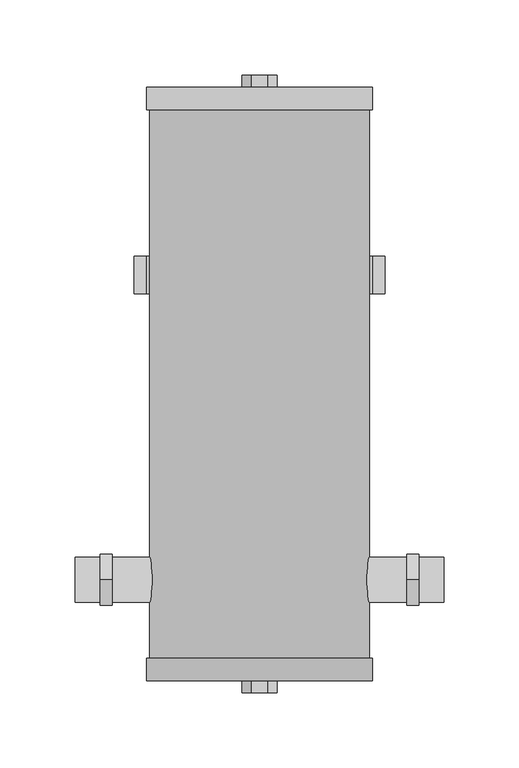
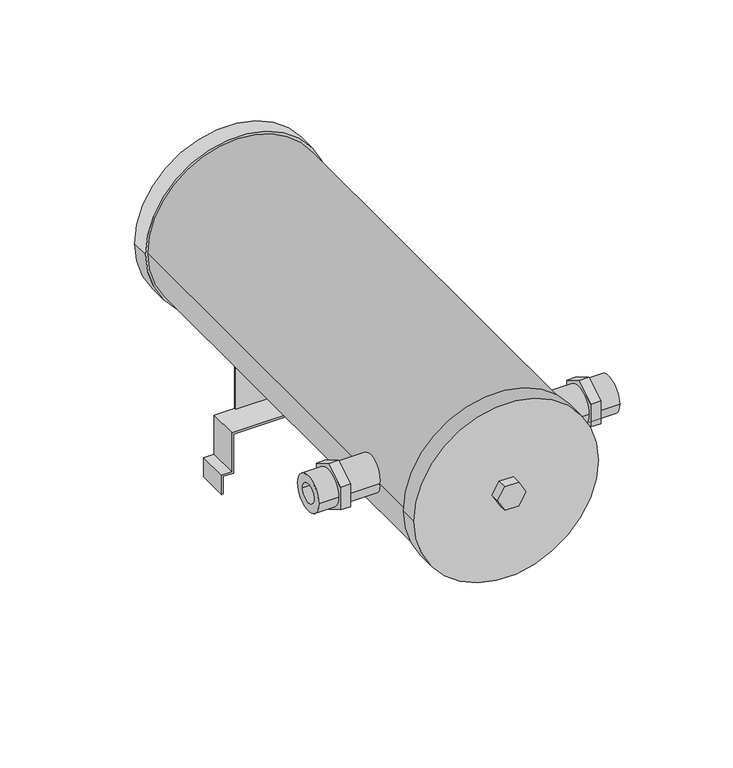
"""IFC4 building model written with IfcOpenShell, lengths in millimetres: proxy geometry, ВЕЗА_ГЕРМИК-Т_ЭПВ230В : ВЕЗА_ГЕРМИК-Т_ЭПВ230В."""

from ifc_helpers import new_model, si_unit, point, frame, frame_2d, origin, place, context, project, spatial, polyline, circle_curve, trimmed, segment, composite_curve, outline, extrude, source, transform, mapped, element, save


def mechanical_equipment_c02479b0(model_context):
    return source(origin(), model_context, "Body", "SweptSolid", [
        extrude(outline(polyline([(-35.0, -73.4905605), (-1.5, -73.4905605), (-1.5, 73.4905605), (-35.0, 73.4905605), (-35.0, 82.0), (-50.0, 82.0), (-50.0, 83.5), (-33.5220792, 83.5), (-33.5220792, 75.0), (0.0, 75.0), (0.0, -75.0), (-33.5220792, -75.0), (-33.5220792, -83.5), (-50.0, -83.5), (-50.0, -82.0), (-35.0, -82.0), (-35.0, -73.4905605)])), frame((0.0, 120.0, 0.0), z_axis=(0.0, 1.0, 0.0), x_axis=(0.0, 0.0, 1.0)), (0.0, 0.0, 1.0), 25.0),
        extrude(outline(composite_curve([segment(polyline([(0.0, 58.4905605), (36.3210082, 58.4905605)]), True, "CONTINUOUS"), segment(trimmed(circle_curve(frame_2d((80.0, 0.0)), 73.0), [point((36.3210082, 58.4905605))], [point((36.3210082, -58.4905605))], True, "CARTESIAN"), True, "CONTINUOUS"), segment(polyline([(36.3210082, -58.4905605), (0.0, -58.4905605), (0.0, 58.4905605)]), True, "CONTINUOUS")], self_intersect=False)), frame((0.0, 143.5, 0.0), z_axis=(0.0, 1.0, 0.0), x_axis=(0.0, 0.0, 1.0)), (0.0, 0.0, 1.0), 1.5),
        extrude(outline(polyline([(-70.0, 99.6451716), (-52.9867823, 89.8225858), (-52.9867823, 70.1774142), (-70.0, 60.3548284), (-87.0132177, 70.1774142), (-87.0132177, 89.8225858), (-70.0, 99.6451716)])), frame((98.0, 0.0, 0.0), z_axis=(1.0, 0.0, 0.0), x_axis=(0.0, 1.0, 0.0)), (0.0, 0.0, 1.0), 8.0),
        extrude(outline(polyline([(-70.0, 99.6451716), (-52.9867823, 89.8225858), (-52.9867823, 70.1774142), (-70.0, 60.3548284), (-87.0132177, 70.1774142), (-87.0132177, 89.8225858), (-70.0, 99.6451716)])), frame((-106.0, 0.0, 0.0), z_axis=(1.0, 0.0, 0.0), x_axis=(0.0, 1.0, 0.0)), (0.0, 0.0, 1.0), 8.0),
        extrude(outline(composite_curve([segment(trimmed(circle_curve(frame_2d((-70.0, 80.0)), 15.0), [point((-85.0, 80.0))], [point((-55.0, 80.0))], False, "CARTESIAN"), True, "CONTINUOUS"), segment(trimmed(circle_curve(frame_2d((-70.0, 80.0)), 15.0), [point((-55.0, 80.0))], [point((-85.0, 80.0))], False, "CARTESIAN"), True, "CONTINUOUS")], self_intersect=False), holes=[composite_curve([segment(trimmed(circle_curve(frame_2d((-70.0, 80.0)), 8.0322911), [point((-78.0322911, 80.0))], [point((-61.9677089, 80.0))], True, "CARTESIAN"), True, "CONTINUOUS"), segment(trimmed(circle_curve(frame_2d((-70.0, 80.0)), 8.0322911), [point((-61.9677089, 80.0))], [point((-78.0322911, 80.0))], True, "CARTESIAN"), True, "CONTINUOUS")], self_intersect=False)]), frame((-122.5, 0.0, 0.0), z_axis=(1.0, 0.0, 0.0), x_axis=(0.0, 1.0, 0.0)), (0.0, 0.0, 1.0), 245.0),
        extrude(outline(polyline([(90.0, -5.7735027), (80.0, -11.5470054), (70.0, -5.7735027), (70.0, 5.7735027), (80.0, 11.5470054), (90.0, 5.7735027), (90.0, -5.7735027)])), frame((0.0, 257.0, 0.0), z_axis=(0.0, 1.0, 0.0), x_axis=(0.0, 0.0, 1.0)), (0.0, 0.0, 1.0), 8.0),
        extrude(outline(polyline([(90.0, -5.7735027), (80.0, -11.5470054), (70.0, -5.7735027), (70.0, 5.7735027), (80.0, 11.5470054), (90.0, 5.7735027), (90.0, -5.7735027)])), frame((0.0, -145.0, 0.0), z_axis=(0.0, 1.0, 0.0), x_axis=(0.0, 0.0, 1.0)), (0.0, 0.0, 1.0), 8.0),
        extrude(outline(composite_curve([segment(trimmed(circle_curve(frame_2d((80.0, 0.0)), 73.0), [point((80.0, 73.0))], [point((80.0, -73.0))], False, "CARTESIAN"), True, "CONTINUOUS"), segment(trimmed(circle_curve(frame_2d((80.0, 0.0)), 73.0), [point((80.0, -73.0))], [point((80.0, 73.0))], False, "CARTESIAN"), True, "CONTINUOUS")], self_intersect=False)), frame((0.0, -122.0, 0.0), z_axis=(0.0, 1.0, 0.0), x_axis=(0.0, 0.0, 1.0)), (0.0, 0.0, 1.0), 364.0),
        extrude(outline(composite_curve([segment(trimmed(circle_curve(frame_2d((80.0, 0.0)), 75.0), [point((80.0, 75.0))], [point((80.0, -75.0))], False, "CARTESIAN"), True, "CONTINUOUS"), segment(trimmed(circle_curve(frame_2d((80.0, 0.0)), 75.0), [point((80.0, -75.0))], [point((80.0, 75.0))], False, "CARTESIAN"), True, "CONTINUOUS")], self_intersect=False)), frame((0.0, 242.0, 0.0), z_axis=(0.0, 1.0, 0.0), x_axis=(0.0, 0.0, 1.0)), (0.0, 0.0, 1.0), 15.0),
        extrude(outline(composite_curve([segment(trimmed(circle_curve(frame_2d((80.0, 0.0)), 75.0), [point((80.0, 75.0))], [point((80.0, -75.0))], False, "CARTESIAN"), True, "CONTINUOUS"), segment(trimmed(circle_curve(frame_2d((80.0, 0.0)), 75.0), [point((80.0, -75.0))], [point((80.0, 75.0))], False, "CARTESIAN"), True, "CONTINUOUS")], self_intersect=False)), frame((0.0, -137.0, 0.0), z_axis=(0.0, 1.0, 0.0), x_axis=(0.0, 0.0, 1.0)), (0.0, 0.0, 1.0), 15.0),
    ])


if __name__ == "__main__":
    model = new_model("IFC4")
    model_context = context("Model", 3, world=origin())
    ifc_project = project(units=[si_unit("LENGTHUNIT", "METRE", prefix="MILLI")], contexts=[model_context])
    site = spatial("IfcSite", under=ifc_project)
    building = spatial("IfcBuilding", under=site)
    placement = place(None, origin())
    mechanical_equipment_shape = mechanical_equipment_c02479b0(model_context)
    element("IfcBuildingElementProxy", 1, Name="ВЕЗА_ГЕРМИК-Т_ЭПВ230В : ВЕЗА_ГЕРМИК-Т_ЭПВ230В", ObjectType="ВЕЗА_ГЕРМИК-Т_ЭПВ230В : ВЕЗА_ГЕРМИК-Т_ЭПВ230В", at=placement, inside=building, context=model_context, shape_type="MappedRepresentation", body=[
        mapped(mechanical_equipment_shape, transform((0.0, 0.0, 0.0), x_axis=(1.0, 0.0, 0.0), y_axis=(0.0, 1.0, 0.0), z_axis=(0.0, 0.0, 1.0))),
    ])
    save(model, "model.ifc")

# Revit data of these elements
# Type "ВЕЗА_ГЕРМИК-Т_ЭПВ230В : ВЕЗА_ГЕРМИК-Т_ЭПВ230В"
#   ВЕЗА_Контакты = "bim@veza.ru"
#   ВЕЗА_Классификатор = ""
#   ADSK_Примечание = "!Не учитывать"
#   ADSK_Позиция = ""
#   ADSK_Наименование краткое = ""
#   ADSK_Наименование = "Взрывозащищенный электропривод ЭПВ"
#   ADSK_Марка = ""
#   ADSK_Комплект = ""
#   ADSK_Код изделия = ""
#   ADSK_Завод-изготовитель = "ООО ''ВЕЗА''"
#   ADSK_Единица измерения = "шт."
#   ADSK_Группирование = ""
#   ВЕЗА_Высота_ручки [instance default] = 37.4 mm
#   ADSK_Напряжение [instance default] = 230 V
#   ADSK_Масса = 0
#   ADSK_Количество = 1
#   упор [instance default] = yes
#   Дополнительная опора [instance default] = yes
#   Корпус = ВЕЗА_сталь нержавеющая
#   Default Elevation = 0
#   Type Comments = ""
#   Manufacturer = ""
# Element 1 (IfcBuildingElementProxy, "ВЕЗА_ГЕРМИК-Т_ЭПВ230В : ВЕЗА_ГЕРМИК-Т_ЭПВ230В")
#   Дополнительная опора = no
#   Materials on its faces: "ВЕЗА_сталь нержавеющая"
# Materials
#   "ВЕЗА_сталь нержавеющая": class "Металл", colour RGB 120 120 120, transparency 0, Description = "Веза_Сталь нержавеющая", Cost = 0
